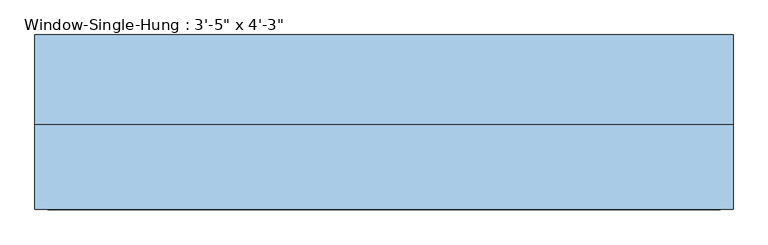
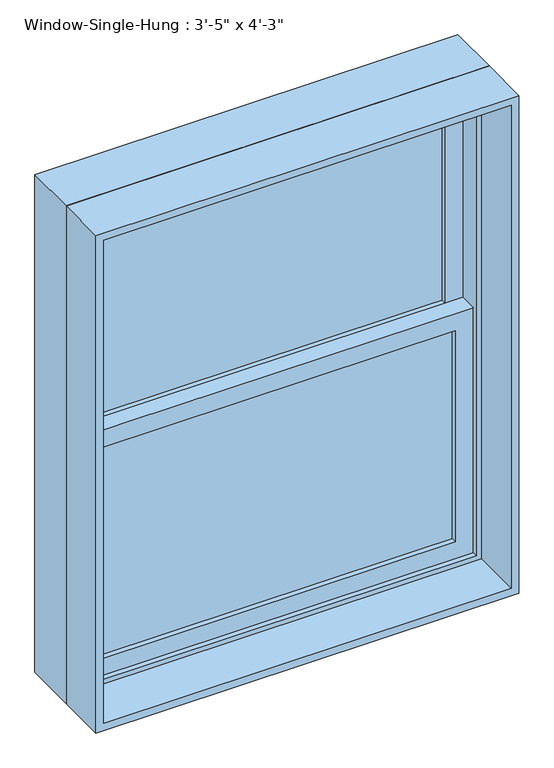
"""IFC4 building model written with IfcOpenShell, lengths in millimetres: window geometry."""

from ifc_helpers import new_model, si_unit, frame, origin, place, context, project, spatial, polyline, outline, extrude, source, transform, mapped, element, save


def window_612ac2e1(model_context):
    return source(origin(), model_context, "Body", "SweptSolid", [
        extrude(outline(polyline([(444.5, 50.8), (444.5, 44.45), (-444.5, 44.45), (-444.5, 50.8), (444.5, 50.8)])), frame((0.0, 0.0, 990.6), z_axis=(0.0, 0.0, 1.0), x_axis=(1.0, 0.0, 0.0)), (0.0, 0.0, 1.0), 549.275),
        extrude(outline(polyline([(-444.5, 38.1), (444.5, 38.1), (444.5, 31.75), (-444.5, 31.75), (-444.5, 38.1)])), frame((0.0, 0.0, 990.6), z_axis=(0.0, 0.0, 1.0), x_axis=(1.0, 0.0, 0.0)), (0.0, 0.0, 1.0), 549.275),
        extrude(outline(polyline([(444.5, 95.25), (444.5, 88.9), (-444.5, 88.9), (-444.5, 95.25), (444.5, 95.25)])), frame((0.0, 0.0, 1584.325), z_axis=(0.0, 0.0, 1.0), x_axis=(1.0, 0.0, 0.0)), (0.0, 0.0, 1.0), 549.275),
        extrude(outline(polyline([(-444.5, 82.55), (444.5, 82.55), (444.5, 76.2), (-444.5, 76.2), (-444.5, 82.55)])), frame((0.0, 0.0, 1584.325), z_axis=(0.0, 0.0, 1.0), x_axis=(1.0, 0.0, 0.0)), (0.0, 0.0, 1.0), 549.275),
        extrude(outline(polyline([(1584.325, -488.95), (946.15, -488.95), (946.15, 488.95), (1584.325, 488.95), (1584.325, -488.95)]), holes=[polyline([(1539.875, 444.5), (990.6, 444.5), (990.6, -444.5), (1539.875, -444.5), (1539.875, 444.5)])]), frame((0.0, 19.05, 0.0), z_axis=(0.0, 1.0, 0.0), x_axis=(0.0, 0.0, 1.0)), (0.0, 0.0, 1.0), 44.45),
        extrude(outline(polyline([(2178.05, -488.95), (1539.875, -488.95), (1539.875, 488.95), (2178.05, 488.95), (2178.05, -488.95)]), holes=[polyline([(2133.6, 444.5), (1584.325, 444.5), (1584.325, -444.5), (2133.6, -444.5), (2133.6, 444.5)])]), frame((0.0, 63.5, 0.0), z_axis=(0.0, 1.0, 0.0), x_axis=(0.0, 0.0, 1.0)), (0.0, 0.0, 1.0), 44.45),
        extrude(outline(polyline([(2209.8, -520.7), (914.4, -520.7), (914.4, 520.7), (2209.8, 520.7), (2209.8, -520.7)]), holes=[polyline([(2178.05, 488.95), (946.15, 488.95), (946.15, -488.95), (2178.05, -488.95), (2178.05, 488.95)])]), frame((0.0, 6.35, 0.0), z_axis=(0.0, 1.0, 0.0), x_axis=(0.0, 0.0, 1.0)), (0.0, 0.0, 1.0), 133.35),
        extrude(outline(polyline([(2209.8, 520.7), (2209.8, -520.7), (914.4, -520.7), (914.4, 520.7), (2209.8, 520.7)]), holes=[polyline([(2190.75, 501.65), (933.45, 501.65), (933.45, -501.65), (2190.75, -501.65), (2190.75, 501.65)])]), frame((0.0, -120.65, 0.0), z_axis=(0.0, 1.0, 0.0), x_axis=(0.0, 0.0, 1.0)), (0.0, 0.0, 1.0), 127.0),
    ])


if __name__ == "__main__":
    model = new_model("IFC4")
    model_context = context("Model", 3, world=origin())
    ifc_project = project(units=[si_unit("LENGTHUNIT", "METRE", prefix="MILLI")], contexts=[model_context])
    site = spatial("IfcSite", under=ifc_project)
    building = spatial("IfcBuilding", under=site)
    placement = place(None, origin())
    window_shape = window_612ac2e1(model_context)
    element("IfcWindow", 1, ObjectType="Window-Single-Hung : 3'-5\" x 4'-3\"", at=placement, inside=building, context=model_context, shape_type="MappedRepresentation", body=[
        mapped(window_shape, transform((0.0, 0.0, 0.0), x_axis=(1.0, 0.0, 0.0), y_axis=(0.0, 1.0, 0.0), z_axis=(0.0, 0.0, 1.0))),
    ])
    save(model, "model.ifc")

# Revit data of these elements
# Type "Window-Single-Hung : 3'-5\" x 4'-3\""
#   Type Mark = "08"
#   Fire Rating = "0.5h"
#   Construction Type Id = "DG-DR"
#   Assembly Code = "B2020100"
#   Analytic Construction = "Double glazing - domestic"
#   Wall Thickness [instance default] = 0' - 6"
#   Window Inset [instance default] = 0' - 0"
#   Visual Light Transmittance = 0.81
#   Thermal Resistance (R) = 0.319569 (m²·K)/W
#   Solar Heat Gain Coefficient = 0.76
#   Muntin Width = 2' - 11"
#   Muntin Height = 1' - 9 5/8"
#   Interior Wall Closure [instance default] = 0' - 1 1/2"
#   Rough Width = 3' - 5 1/2"
#   Rough Height = 4' - 3 1/2"
#   Frame Extension [instance default] = 0' - 1 1/4"
#   Exterior Wall Closure [instance default] = 0' - 0 1/2"
#   Extension Jamb [instance default] = 0' - 1 1/2"
#   Heat Transfer Coefficient (U) = 3.12929 W/(m²·K)
#   Height = 4' - 3"
#   Width = 3' - 5"
#   Top Muntin Visibility = no
#   Indicator Visibility = no
#   Extension Jamb Visibility [instance default] = yes
#   Interior Trim Visibility [instance default] = yes
#   Exterior Trim Visibility [instance default] = yes
#   Bottom Muntin Visibility = no
#   Muntin Pattern = Muntin Pattern_2x2 : Muntin Pattern_2x2
#   Interior Trim Material = 1X WOOD COMPOSITE TRIM
#   Interior Trim = Trim-Window-Interior-Flat : Picture Frame
#   Exterior Trim Material = 1X WOOD COMPOSITE TRIM
#   Exterior Trim = Trim-Window-Exterior-Flat : with Sill
#   Glass Panel Material = NEW DOUBLE HUNG WINDOWS (TYP.)
#   Exterior Frame Material = 1X WOOD COMPOSITE TRIM
#   Interior Frame Material = 1X WOOD COMPOSITE TRIM
#   Wall Closure = (empty or 0)
# Element 1 (IfcWindow, "Window-Single-Hung : 3'-5\" x 4'-3\"")
#   Wall Thickness = 0' - 9 1/2"
#   Extension Jamb = 0' - 5"
#   Materials on its faces: "1X WOOD COMPOSITE TRIM", "NEW DOUBLE HUNG WINDOWS (TYP.)"
# Materials
#   "1X WOOD COMPOSITE TRIM": class "Generic", colour RGB 88 61 61, transparency 0, Cost = 0
#   "NEW DOUBLE HUNG WINDOWS (TYP.)": class "Glass", colour RGB 218 227 224, transparency 0.85, Description = "Soda Lime Glass", Cost = 0
